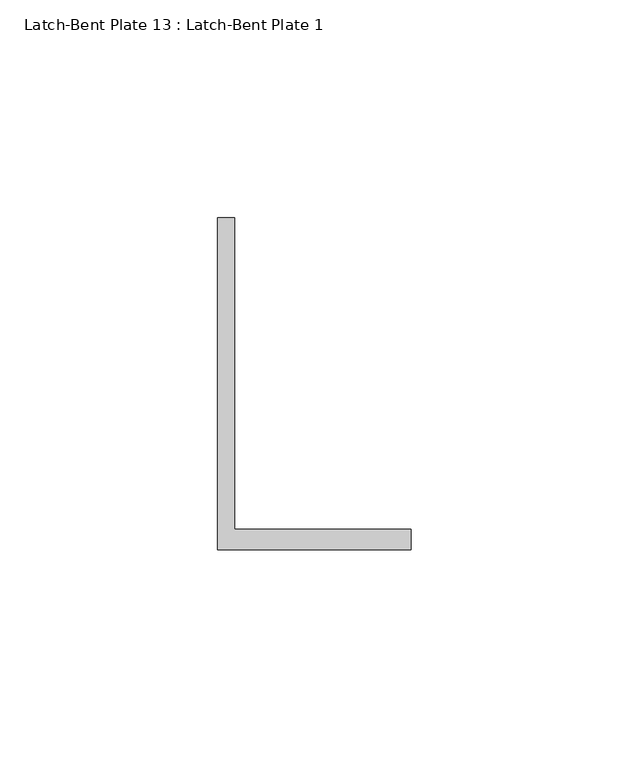
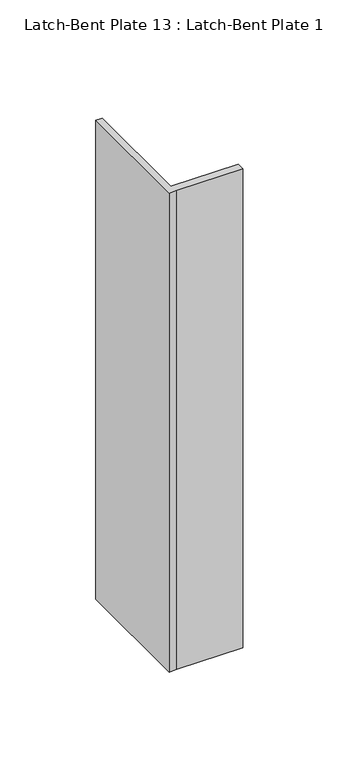
"""IFC4 building model written with IfcOpenShell, lengths in millimetres: proxy geometry, Latch-Bent Plate 13 : Latch-Bent Plate 1."""

from ifc_helpers import new_model, si_unit, frame, origin, place, context, project, spatial, polyline, outline, extrude, source, transform, mapped, element, save


def latch_bent_plate_13_latch_bent_plate_1_8bdba4d9(model_context):
    return source(origin(), model_context, "Body", "SweptSolid", [
        extrude(outline(polyline([(587327.0060739, -535201.5663841), (587322.2435739, -535201.5663841), (587322.2435739, -535125.3663841), (587326.1141748, -535125.3663841), (587326.1141748, -535196.8038841), (587366.6808739, -535196.8038841), (587366.6808739, -535201.5663841), (587327.0060739, -535201.5663841)])), frame((0.0, 0.0, 50.8), z_axis=(0.0, 0.0, 1.0), x_axis=(1.0, 0.0, 0.0)), (0.0, 0.0, 1.0), 304.8),
    ])


if __name__ == "__main__":
    model = new_model("IFC4")
    model_context = context("Model", 3, world=origin())
    ifc_project = project(units=[si_unit("LENGTHUNIT", "METRE", prefix="MILLI")], contexts=[model_context])
    site = spatial("IfcSite", under=ifc_project)
    building = spatial("IfcBuilding", under=site)
    placement = place(None, origin())
    latch_bent_plate_13_latch_bent_plate_1_shape = latch_bent_plate_13_latch_bent_plate_1_8bdba4d9(model_context)
    element("IfcBuildingElementProxy", 1, Name="Latch-Bent Plate 13 : Latch-Bent Plate 1", ObjectType="Latch-Bent Plate 13 : Latch-Bent Plate 1", at=placement, inside=building, context=model_context, shape_type="MappedRepresentation", body=[
        mapped(latch_bent_plate_13_latch_bent_plate_1_shape, transform((0.0, 0.0, 0.0), x_axis=(1.0, 0.0, 0.0), y_axis=(0.0, 1.0, 0.0), z_axis=(0.0, 0.0, 1.0))),
    ])
    save(model, "model.ifc")

# Revit data of these elements
# Element 1 (IfcBuildingElementProxy, "Latch-Bent Plate 13 : Latch-Bent Plate 1")
#   Materials on its faces: "GALV. GATE LATCH"
# Materials
#   "GALV. GATE LATCH": class "Metal", colour RGB 189 187 185, transparency 0, Description = "Carbon steel", Cost = 0
